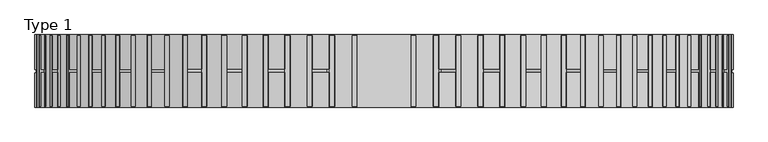
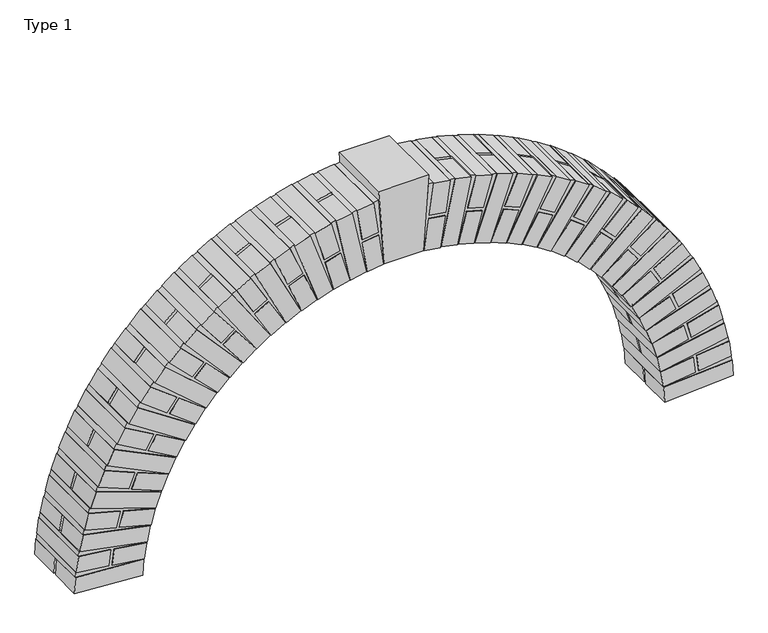
"""IFC4 building model written with IfcOpenShell, lengths in millimetres: proxy geometry, 00_GM_toog : Type 1."""

from ifc_helpers import new_model, si_unit, frame, origin, place, context, project, spatial, polyline, outline, extrude, source, transform, mapped, element, save


def type_1_de08efeb(model_context):
    return source(origin(), model_context, "Body", "SweptSolid", [
        extrude(outline(polyline([(-41.1694034, 158.0337642), (-39.7015699, 142.0396534), (-138.7087275, 127.9832407), (-131.6805212, 78.4796619), (-32.6733636, 92.5360745), (-30.4140828, 76.622699), (-231.7563983, 61.2874572), (-232.3621237, 64.1855221), (-141.8118024, 77.0412864), (-148.8400087, 126.5448652), (-241.2763519, 113.4213355), (-241.8346853, 116.0926555), (-41.1694034, 158.0337642)])), frame((0.0, 2.5, 0.0), z_axis=(0.0, 1.0, 0.0), x_axis=(0.0, 0.0, 1.0)), (0.0, 0.0, 1.0), 205.0),
        extrude(outline(polyline([(0.0, 50.0), (210.0, 50.0), (210.0, 0.0), (0.0, 0.0), (0.0, 50.0)])), frame((78.4796619, 210.0, -131.6805212), z_axis=(0.14056412625055034, 0.0, 0.9900715764082006), x_axis=(0.0, -1.0, 0.0)), (0.0, 0.0, 1.0), 100.0),
        extrude(outline(polyline([(0.0, 50.0), (210.0, 50.0), (210.0, 0.0), (0.0, 0.0), (0.0, 50.0)])), frame((62.9848738, 210.0, -240.81896), z_axis=(0.14056412625055034, 0.0, 0.9900715764082006), x_axis=(0.0, -1.0, 0.0)), (0.0, 0.0, 1.0), 100.0),
        extrude(outline(polyline([(210.0, 50.0000001), (210.0, 0.0), (110.0, 0.0), (110.0, 50.0000001), (210.0, 50.0000001)])), frame((164.0124098, 0.0, -256.956928), z_axis=(0.2045892845565526, 0.0, 0.9788479067989255), x_axis=(0.0, 1.0, 0.0)), (0.0, 0.0, 1.0), 210.0),
        extrude(outline(polyline([(100.0, 50.0000001), (100.0, 0.0), (0.0, 0.0), (0.0, 50.0000001), (100.0, 50.0000001)])), frame((164.0124098, 0.0, -256.956928), z_axis=(0.2045892845565526, 0.0, 0.9788479067989255), x_axis=(0.0, 1.0, 0.0)), (0.0, 0.0, 1.0), 210.0),
        extrude(outline(polyline([(-70.1056799, 286.4239748), (-66.5764443, 270.7551966), (-162.925286, 243.9801952), (-149.5377853, 195.8057743), (-53.1889436, 222.5807757), (-48.8854098, 207.0946701), (-246.5397389, 165.7828815), (-247.5161135, 168.5779444), (-159.3970443, 193.0659212), (-172.784545, 241.2403421), (-262.7389968, 216.2423189), (-263.6389798, 218.8186958), (-70.1056799, 286.4239748)])), frame((0.0, 2.5, 0.0), z_axis=(0.0, 1.0, 0.0), x_axis=(0.0, 0.0, 1.0)), (0.0, 0.0, 1.0), 205.0),
        extrude(outline(polyline([(0.0, 50.0), (210.0, 50.0), (210.0, 0.0), (0.0, 0.0), (0.0, 50.0)])), frame((195.8057743, 210.0, -149.5377853), z_axis=(0.26775001392461106, 0.0, 0.9634884171817379), x_axis=(0.0, -1.0, 0.0)), (0.0, 0.0, 1.0), 100.0),
        extrude(outline(polyline([(0.0, 50.0), (210.0, 50.0), (210.0, 0.0), (0.0, 0.0), (0.0, 50.0)])), frame((166.2909198, 210.0, -255.745886), z_axis=(0.26775001392461106, 0.0, 0.9634884171817379), x_axis=(0.0, -1.0, 0.0)), (0.0, 0.0, 1.0), 100.0),
        extrude(outline(polyline([(210.0, 50.0), (210.0, 0.0), (110.0, 0.0), (110.0, 50.0), (210.0, 50.0)])), frame((264.3731909, 0.0, -284.8468332), z_axis=(0.3297794481680561, 0.0, 0.9440580043439982), x_axis=(0.0, 1.0, 0.0)), (0.0, 0.0, 1.0), 210.0),
        extrude(outline(polyline([(100.0, 50.0), (100.0, 0.0), (0.0, 0.0), (0.0, 50.0), (100.0, 50.0)])), frame((264.3731909, 0.0, -284.8468332), z_axis=(0.3297794481680561, 0.0, 0.9440580043439982), x_axis=(0.0, 1.0, 0.0)), (0.0, 0.0, 1.0), 210.0),
        extrude(outline(polyline([(-115.4447373, 409.978514), (-109.9136834, 394.899603), (-201.9775599, 355.8580528), (-182.4567849, 309.8261146), (-90.3929083, 348.8676647), (-84.1177777, 334.0702796), (-274.7471392, 267.4794077), (-276.077679, 270.1242796), (-191.8775686, 305.8310406), (-211.3983437, 351.8629788), (-297.3522109, 315.4125018), (-298.5786492, 317.8504387), (-115.4447373, 409.978514)])), frame((0.0, 2.5, 0.0), z_axis=(0.0, 1.0, 0.0), x_axis=(0.0, 0.0, 1.0)), (0.0, 0.0, 1.0), 205.0),
        extrude(outline(polyline([(0.0, 49.9999999), (210.0, 49.9999999), (210.0, 0.0), (0.0, 0.0), (0.0, 49.9999999)])), frame((309.8261146, 210.0, -182.4567849), z_axis=(0.39041550103890255, 0.0, 0.9206387655038988), x_axis=(0.0, -1.0, 0.0)), (0.0, 0.0, 1.0), 100.0),
        extrude(outline(polyline([(0.0, 49.9999999), (210.0, 49.9999999), (210.0, 0.0), (0.0, 0.0), (0.0, 49.9999999)])), frame((266.7894905, 210.0, -283.9414452), z_axis=(0.39041550103890255, 0.0, 0.9206387655038988), x_axis=(0.0, -1.0, 0.0)), (0.0, 0.0, 1.0), 100.0),
        extrude(outline(polyline([(210.0, 50.0), (210.0, 0.0), (110.0, 0.0), (110.0, 50.0), (210.0, 50.0)])), frame((360.2705822, 0.0, -325.5140628), z_axis=(0.4494019735925478, 0.0, 0.8933296514339615), x_axis=(0.0, 1.0, 0.0)), (0.0, 0.0, 1.0), 210.0),
        extrude(outline(polyline([(100.0, 50.0), (100.0, 0.0), (0.0, 0.0), (0.0, 50.0), (100.0, 50.0)])), frame((360.2705822, 0.0, -325.5140628), z_axis=(0.4494019735925478, 0.0, 0.8933296514339615), x_axis=(0.0, 1.0, 0.0)), (0.0, 0.0, 1.0), 210.0),
        extrude(outline(polyline([(-176.4211202, 526.6114211), (-168.9816283, 512.3769532), (-255.2062332, 461.7279895), (-229.8817513, 418.6156871), (-143.6571465, 469.2646507), (-135.5163616, 455.4058092), (-315.9023763, 364.6601019), (-317.5646179, 367.1101298), (-238.7050095, 413.4328407), (-264.0294914, 456.5451431), (-344.5316223, 409.2576025), (-346.0638099, 411.5159399), (-176.4211202, 526.6114211)])), frame((0.0, 2.5, 0.0), z_axis=(0.0, 1.0, 0.0), x_axis=(0.0, 0.0, 1.0)), (0.0, 0.0, 1.0), 205.0),
        extrude(outline(polyline([(0.0, 50.0), (210.0, 50.0), (210.0, 0.0), (0.0, 0.0), (0.0, 50.0)])), frame((418.6156871, 210.0, -229.8817513), z_axis=(0.5064896366773486, 0.0, 0.8622460483750839), x_axis=(0.0, -1.0, 0.0)), (0.0, 0.0, 1.0), 100.0),
        extrude(outline(polyline([(0.0, 50.0), (210.0, 50.0), (210.0, 0.0), (0.0, 0.0), (0.0, 50.0)])), frame((362.783877, 210.0, -324.9296144), z_axis=(0.5064896366773486, 0.0, 0.8622460483750839), x_axis=(0.0, -1.0, 0.0)), (0.0, 0.0, 1.0), 100.0),
        extrude(outline(polyline([(210.0, 50.0), (210.0, 0.0), (110.0, 0.0), (110.0, 50.0), (210.0, 50.0)])), frame((450.085556, 0.0, -378.2720354), z_axis=(0.5614372839756181, 0.0, 0.8275192905075271), x_axis=(0.0, 1.0, 0.0)), (0.0, 0.0, 1.0), 210.0),
        extrude(outline(polyline([(100.0, 50.0), (100.0, 0.0), (0.0, 0.0), (0.0, 50.0), (100.0, 50.0)])), frame((450.085556, 0.0, -378.2720354), z_axis=(0.5614372839756181, 0.0, 0.8275192905075271), x_axis=(0.0, 1.0, 0.0)), (0.0, 0.0, 1.0), 210.0),
        extrude(outline(polyline([(-252.0053697, 634.3535926), (-242.7830401, 621.2038872), (-321.7126506, 559.802612), (-291.012013, 520.3378068), (-212.0824025, 581.7390819), (-202.2134034, 569.0527614), (-369.3106297, 455.6842709), (-371.2765096, 457.8980911), (-299.0887834, 514.0546895), (-329.7894209, 553.5194948), (-403.4807049, 496.1932421), (-405.2927741, 498.2338527), (-252.0053697, 634.3535926)])), frame((0.0, 2.5, 0.0), z_axis=(0.0, 1.0, 0.0), x_axis=(0.0, 0.0, 1.0)), (0.0, 0.0, 1.0), 205.0),
        extrude(outline(polyline([(0.0, 50.0), (210.0, 50.0), (210.0, 0.0), (0.0, 0.0), (0.0, 50.0)])), frame((520.3378068, 210.0, -291.012013), z_axis=(0.6140127511464796, 0.0, 0.7892961050388704), x_axis=(0.0, -1.0, 0.0)), (0.0, 0.0, 1.0), 100.0),
        extrude(outline(polyline([(0.0, 49.9999999), (210.0, 49.9999999), (210.0, 0.0), (0.0, 0.0), (0.0, 49.9999999)])), frame((452.6534144, 210.0, -378.0183939), z_axis=(0.6140127511464796, 0.0, 0.7892961050388704), x_axis=(0.0, -1.0, 0.0)), (0.0, 0.0, 1.0), 100.0),
        extrude(outline(polyline([(210.0, 50.0), (210.0, 0.0), (110.0, 0.0), (110.0, 50.0), (210.0, 50.0)])), frame((532.3017739, 0.0, -442.2300429), z_axis=(0.663993896764768, 0.0, 0.7477379922533953), x_axis=(0.0, 1.0, 0.0)), (0.0, 0.0, 1.0), 210.0),
        extrude(outline(polyline([(100.0, 50.0), (100.0, 0.0), (0.0, 0.0), (0.0, 50.0), (100.0, 50.0)])), frame((532.3017739, 0.0, -442.2300429), z_axis=(0.663993896764768, 0.0, 0.7477379922533953), x_axis=(0.0, 1.0, 0.0)), (0.0, 0.0, 1.0), 210.0),
        extrude(outline(polyline([(-340.9214032, 731.3860267), (-330.0719357, 719.5430891), (-400.37399, 648.426135), (-364.8155129, 613.2751079), (-294.5134586, 684.3920619), (-283.0828629, 673.0924447), (-434.0702126, 539.0151613), (-436.306541, 540.9553981), (-372.009436, 605.997797), (-407.5679131, 641.1488242), (-473.2042264, 574.7516936), (-475.2655843, 576.5401261), (-340.9214032, 731.3860267)])), frame((0.0, 2.5, 0.0), z_axis=(0.0, 1.0, 0.0), x_axis=(0.0, 0.0, 1.0)), (0.0, 0.0, 1.0), 205.0),
        extrude(outline(polyline([(0.0, 100.0), (210.0, 100.0), (210.0, 0.0), (0.0, 0.0), (0.0, 100.0)])), frame((648.426135, 210.0, -400.37399), z_axis=(-0.7030205431424774, 0.0, 0.7111695409110659), x_axis=(0.0, -1.0, 0.0)), (0.0, 0.0, 1.0), 50.0),
        extrude(outline(polyline([(0.0, 100.0), (210.0, 100.0), (210.0, 0.0), (0.0, 0.0), (0.0, 100.0)])), frame((570.0318701, 210.0, -477.8699674), z_axis=(-0.7030205431424774, 0.0, 0.7111695409110659), x_axis=(0.0, -1.0, 0.0)), (0.0, 0.0, 1.0), 50.0),
        extrude(outline(polyline([(0.0, 100.0), (210.0, 100.0), (210.0, 0.0), (0.0, 0.0), (0.0, 100.0)])), frame((605.5311866, 110.0, -516.3082875), z_axis=(-0.655332697498948, 0.0, 0.755340357447391), x_axis=(0.755340357447391, 0.0, 0.655332697498948)), (0.0, 0.0, 1.0), 50.0),
        extrude(outline(polyline([(0.0, 100.0), (210.0, 100.0), (210.0, 0.0), (0.0, 0.0), (0.0, 100.0)])), frame((605.5311866, 0.0, -516.3082875), z_axis=(-0.655332697498948, 0.0, 0.755340357447391), x_axis=(0.755340357447391, 0.0, 0.655332697498948)), (0.0, 0.0, 1.0), 50.0),
        extrude(outline(polyline([(-441.6680589, 816.0705332), (-429.3746242, 805.7343067), (-489.8622187, 726.1023351), (-450.0462329, 695.8585378), (-389.5586384, 775.4905094), (-376.7594277, 765.7683658), (-509.0877943, 613.2459049), (-511.5568156, 614.8798014), (-456.2358544, 687.7098957), (-496.0518402, 717.9536929), (-552.5250506, 643.6066616), (-554.8008954, 645.1127218), (-441.6680589, 816.0705332)])), frame((0.0, 2.5, 0.0), z_axis=(0.0, 1.0, 0.0), x_axis=(0.0, 0.0, 1.0)), (0.0, 0.0, 1.0), 205.0),
        extrude(outline(polyline([(0.0, 99.9999999), (210.0, 99.9999999), (210.0, 0.0), (0.0, 0.0), (0.0, 99.9999999)])), frame((726.1023351, 210.0, -489.8622187), z_axis=(-0.6048759456103062, 0.0, 0.7963197162082813), x_axis=(0.0, -1.0, 0.0)), (0.0, 0.0, 1.0), 50.0),
        extrude(outline(polyline([(0.0, 100.0), (210.0, 100.0), (210.0, 0.0), (0.0, 0.0), (0.0, 100.0)])), frame((638.3217213, 210.0, -556.5394348), z_axis=(-0.6048759456103062, 0.0, 0.7963197162082813), x_axis=(0.0, -1.0, 0.0)), (0.0, 0.0, 1.0), 50.0),
        extrude(outline(polyline([(0.0, 100.0), (210.0000001, 100.0), (210.0000001, 0.0), (0.0, 0.0), (0.0, 100.0)])), frame((668.537468, 110.0, -599.2561127), z_axis=(-0.5518634769235881, 0.0, 0.8339344715490591), x_axis=(0.8339344715490591, 0.0, 0.5518634769235881)), (0.0, 0.0, 1.0), 50.0),
        extrude(outline(polyline([(0.0, 100.0), (210.0000001, 100.0), (210.0000001, 0.0), (0.0, 0.0), (0.0, 100.0)])), frame((668.537468, 0.0, -599.2561127), z_axis=(-0.5518634769235881, 0.0, 0.8339344715490591), x_axis=(0.8339344715490591, 0.0, 0.5518634769235881)), (0.0, 0.0, 1.0), 50.0),
        extrude(outline(polyline([(-552.5444398, 886.9773907), (-539.0145868, 878.322381), (-588.6665147, 791.5198116), (-545.26523, 766.6938476), (-495.6133021, 853.496417), (-481.6615645, 845.5158852), (-593.0968596, 677.1232704), (-595.7568893, 678.4232417), (-550.346051, 757.811447), (-593.7473357, 782.637411), (-640.1040109, 701.5956733), (-642.5559196, 702.7939348), (-552.5444398, 886.9773907)])), frame((0.0, 2.5, 0.0), z_axis=(0.0, 1.0, 0.0), x_axis=(0.0, 0.0, 1.0)), (0.0, 0.0, 1.0), 205.0),
        extrude(outline(polyline([(0.0, 100.0), (210.0, 100.0), (210.0, 0.0), (0.0, 0.0), (0.0, 100.0)])), frame((791.5198116, 210.0, -588.6665147), z_axis=(-0.4965192792791466, 0.0, 0.8680256939193199), x_axis=(0.0, -1.0, 0.0)), (0.0, 0.0, 1.0), 50.0),
        extrude(outline(polyline([(0.0, 100.0), (210.0, 100.0), (210.0, 0.0), (0.0, 0.0), (0.0, 100.0)])), frame((695.8348416, 210.0, -643.3992636), z_axis=(-0.4965192792791466, 0.0, 0.8680256939193199), x_axis=(0.0, -1.0, 0.0)), (0.0, 0.0, 1.0), 50.0),
        extrude(outline(polyline([(0.0, 100.0), (210.0, 100.0), (210.0, 0.0), (0.0, 0.0), (0.0, 100.0)])), frame((720.2568887, 110.0, -689.6731173), z_axis=(-0.4390771925190386, 0.0, 0.898449341370786), x_axis=(0.898449341370786, 0.0, 0.4390771925190386)), (0.0, 0.0, 1.0), 50.0),
        extrude(outline(polyline([(0.0, 100.0), (210.0, 100.0), (210.0, 0.0), (0.0, 0.0), (0.0, 100.0)])), frame((720.2568887, 0.0, -689.6731173), z_axis=(-0.4390771925190386, 0.0, 0.898449341370786), x_axis=(0.898449341370786, 0.0, 0.4390771925190386)), (0.0, 0.0, 1.0), 50.0),
        extrude(outline(polyline([(-671.6786294, 942.9094849), (-657.1407815, 936.0818137), (-695.1187735, 843.5741269), (-648.8649301, 824.5851308), (-610.8869381, 917.0928176), (-596.0182196, 910.9886322), (-684.6790905, 729.5688217), (-687.4852197, 730.5129205), (-652.7511715, 815.1189325), (-699.0050149, 834.1079286), (-734.4625191, 747.7397054), (-737.0490965, 748.6099379), (-671.6786294, 942.9094849)])), frame((0.0, 2.5, 0.0), z_axis=(0.0, 1.0, 0.0), x_axis=(0.0, 0.0, 1.0)), (0.0, 0.0, 1.0), 205.0),
        extrude(outline(polyline([(0.0, 100.0), (210.0, 100.0), (210.0, 0.0), (0.0, 0.0), (0.0, 100.0)])), frame((843.5741269, 210.0, -695.1187735), z_axis=(-0.3797799204689407, 0.0, 0.9250768681621031), x_axis=(0.0, -1.0, 0.0)), (0.0, 0.0, 1.0), 50.0),
        extrude(outline(polyline([(0.0, 100.0), (210.0, 100.0), (210.0, 0.0), (0.0, 0.0), (0.0, 100.0)])), frame((741.6002418, 210.0, -736.983007), z_axis=(-0.3797799204689407, 0.0, 0.9250768681621031), x_axis=(0.0, -1.0, 0.0)), (0.0, 0.0, 1.0), 50.0),
        extrude(outline(polyline([(0.0, 100.0), (210.0, 100.0), (210.0, 0.0), (0.0, 0.0), (0.0, 100.0)])), frame((759.8162739, 110.0, -786.0327989), z_axis=(-0.31887800546790185, 0.0, 0.947795767889271), x_axis=(0.947795767889271, 0.0, 0.31887800546790185)), (0.0, 0.0, 1.0), 50.0),
        extrude(outline(polyline([(0.0, 100.0), (210.0, 100.0), (210.0, 0.0), (0.0, 0.0), (0.0, 100.0)])), frame((759.8162739, 0.0, -786.0327989), z_axis=(-0.31887800546790185, 0.0, 0.947795767889271), x_axis=(0.947795767889271, 0.0, 0.31887800546790185)), (0.0, 0.0, 1.0), 50.0),
        extrude(outline(polyline([(-797.0592953, 982.922519), (-781.7588937, 978.0374573), (-807.4217707, 881.3864524), (-759.0962683, 868.5550139), (-733.4333913, 965.2060188), (-717.8987192, 961.0812362), (-782.2883121, 769.697125), (-785.1931651, 770.2694122), (-761.722319, 858.664835), (-810.0478215, 871.4962734), (-834.0075286, 781.2597121), (-836.6851057, 781.7872235), (-797.0592953, 982.922519)])), frame((0.0, 2.5, 0.0), z_axis=(0.0, 1.0, 0.0), x_axis=(0.0, 0.0, 1.0)), (0.0, 0.0, 1.0), 205.0),
        extrude(outline(polyline([(0.0, 100.0), (210.0, 100.0), (210.0, 0.0), (0.0, 0.0), (0.0, 100.0)])), frame((881.3864524, 210.0, -807.4217707), z_axis=(-0.25662876977901194, 0.0, 0.9665100488467313), x_axis=(0.0, -1.0, 0.0)), (0.0, 0.0, 1.0), 50.0),
        extrude(outline(polyline([(0.0, 99.9999999), (210.0, 99.9999999), (210.0, 0.0), (0.0, 0.0), (0.0, 99.9999999)])), frame((774.8452686, 210.0, -835.7106985), z_axis=(-0.25662876977901194, 0.0, 0.9665100488467313), x_axis=(0.0, -1.0, 0.0)), (0.0, 0.0, 1.0), 50.0),
        extrude(outline(polyline([(0.0, 100.0), (210.0, 100.0), (210.0, 0.0), (0.0, 0.0), (0.0, 100.0)])), frame((786.5477461, 110.0, -886.7083253), z_axis=(-0.19329522835345544, 0.0, 0.9811406396107469), x_axis=(0.9811406396107469, 0.0, 0.19329522835345544)), (0.0, 0.0, 1.0), 50.0),
        extrude(outline(polyline([(0.0, 100.0), (210.0, 100.0), (210.0, 0.0), (0.0, 0.0), (0.0, 100.0)])), frame((786.5477461, 0.0, -886.7083253), z_axis=(-0.19329522835345544, 0.0, 0.9811406396107469), x_axis=(0.9811406396107469, 0.0, 0.19329522835345544)), (0.0, 0.0, 1.0), 50.0),
        extrude(outline(polyline([(-926.5696466, 1006.3409563), (-910.7650067, 1003.4809782), (-923.6795044, 904.3184059), (-874.0982183, 897.861157), (-861.1837205, 997.0237294), (-845.2453653, 994.947988), (-884.2765962, 796.8306977), (-887.2311307, 797.0215114), (-875.419743, 887.7139725), (-925.0010292, 894.1712214), (-937.0584296, 801.5897779), (-939.781801, 801.7656623), (-926.5696466, 1006.3409563)])), frame((0.0, 2.5, 0.0), z_axis=(0.0, 1.0, 0.0), x_axis=(0.0, 0.0, 1.0)), (0.0, 0.0, 1.0), 205.0),
        extrude(outline(polyline([(0.0, 100.0), (210.0, 100.0), (210.0, 0.0), (0.0, 0.0), (0.0, 100.0)])), frame((904.3184059, 210.0, -923.6795044), z_axis=(-0.12914497754199947, 0.0, 0.9916257231313015), x_axis=(0.0, -1.0, 0.0)), (0.0, 0.0, 1.0), 50.0),
        extrude(outline(polyline([(0.0, 100.0000001), (210.0, 100.0000001), (210.0, 0.0), (0.0, 0.0), (0.0, 100.0000001)])), frame((795.008649, 210.0, -937.9155269), z_axis=(-0.12914497754199947, 0.0, 0.9916257231313015), x_axis=(0.0, -1.0, 0.0)), (0.0, 0.0, 1.0), 50.0),
        extrude(outline(polyline([(0.0, 100.0), (210.0, 100.0), (210.0, 0.0), (0.0, 0.0), (0.0, 100.0)])), frame((800.0, 110.0, -990.0), z_axis=(-0.06444906444906115, 0.0, 0.9979209979209982), x_axis=(0.9979209979209982, 0.0, 0.06444906444906115)), (0.0, 0.0, 1.0), 50.0),
        extrude(outline(polyline([(0.0, 100.0), (210.0, 100.0), (210.0, 0.0), (0.0, 0.0), (0.0, 100.0)])), frame((800.0, 0.0, -990.0), z_axis=(-0.06444906444906115, 0.0, 0.9979209979209982), x_axis=(0.9979209979209982, 0.0, 0.06444906444906115)), (0.0, 0.0, 1.0), 50.0),
        extrude(outline(polyline([(-41.1694034, -158.0337642), (-241.8346853, -116.0926555), (-241.2763519, -113.4213355), (-148.8400087, -126.5448652), (-141.8118024, -77.0412864), (-232.3621237, -64.1855221), (-231.7563983, -61.2874572), (-30.4140828, -76.622699), (-32.6733636, -92.5360745), (-131.6805212, -78.4796619), (-138.7087275, -127.9832407), (-39.7015699, -142.0396534), (-41.1694034, -158.0337642)])), frame((0.0, 2.5, 0.0), z_axis=(0.0, 1.0, 0.0), x_axis=(0.0, 0.0, 1.0)), (0.0, 0.0, 1.0), 205.0),
        extrude(outline(polyline([(0.0, -50.0), (0.0, 0.0), (210.0, 0.0), (210.0, -50.0), (0.0, -50.0)])), frame((-78.4796619, 210.0, -131.6805212), z_axis=(-0.14056412625055034, 0.0, 0.9900715764082006), x_axis=(0.0, -1.0, 0.0)), (0.0, 0.0, 1.0), 100.0),
        extrude(outline(polyline([(0.0, -50.0), (0.0, 0.0), (210.0, 0.0), (210.0, -50.0), (0.0, -50.0)])), frame((-62.9848738, 210.0, -240.81896), z_axis=(-0.14056412625055034, 0.0, 0.9900715764082006), x_axis=(0.0, -1.0, 0.0)), (0.0, 0.0, 1.0), 100.0),
        extrude(outline(polyline([(210.0, -50.0000001), (110.0, -50.0000001), (110.0, 0.0), (210.0, 0.0), (210.0, -50.0000001)])), frame((-164.0124098, 0.0, -256.956928), z_axis=(-0.2045892845565526, 0.0, 0.9788479067989255), x_axis=(0.0, 1.0, 0.0)), (0.0, 0.0, 1.0), 210.0),
        extrude(outline(polyline([(100.0, -50.0000001), (0.0, -50.0000001), (0.0, 0.0), (100.0, 0.0), (100.0, -50.0000001)])), frame((-164.0124098, 0.0, -256.956928), z_axis=(-0.2045892845565526, 0.0, 0.9788479067989255), x_axis=(0.0, 1.0, 0.0)), (0.0, 0.0, 1.0), 210.0),
        extrude(outline(polyline([(-70.1056799, -286.4239748), (-263.6389798, -218.8186958), (-262.7389968, -216.2423189), (-172.784545, -241.2403421), (-159.3970443, -193.0659212), (-247.5161135, -168.5779444), (-246.5397389, -165.7828815), (-48.8854098, -207.0946701), (-53.1889436, -222.5807757), (-149.5377853, -195.8057743), (-162.925286, -243.9801952), (-66.5764443, -270.7551966), (-70.1056799, -286.4239748)])), frame((0.0, 2.5, 0.0), z_axis=(0.0, 1.0, 0.0), x_axis=(0.0, 0.0, 1.0)), (0.0, 0.0, 1.0), 205.0),
        extrude(outline(polyline([(0.0, -50.0), (0.0, 0.0), (210.0, 0.0), (210.0, -50.0), (0.0, -50.0)])), frame((-195.8057743, 210.0, -149.5377853), z_axis=(-0.26775001392461106, 0.0, 0.9634884171817379), x_axis=(0.0, -1.0, 0.0)), (0.0, 0.0, 1.0), 100.0),
        extrude(outline(polyline([(0.0, -50.0), (0.0, 0.0), (210.0, 0.0), (210.0, -50.0), (0.0, -50.0)])), frame((-166.2909198, 210.0, -255.745886), z_axis=(-0.26775001392461106, 0.0, 0.9634884171817379), x_axis=(0.0, -1.0, 0.0)), (0.0, 0.0, 1.0), 100.0),
        extrude(outline(polyline([(210.0, -50.0), (110.0, -50.0), (110.0, 0.0), (210.0, 0.0), (210.0, -50.0)])), frame((-264.3731909, 0.0, -284.8468332), z_axis=(-0.3297794481680561, 0.0, 0.9440580043439982), x_axis=(0.0, 1.0, 0.0)), (0.0, 0.0, 1.0), 210.0),
        extrude(outline(polyline([(100.0, -50.0), (0.0, -50.0), (0.0, 0.0), (100.0, 0.0), (100.0, -50.0)])), frame((-264.3731909, 0.0, -284.8468332), z_axis=(-0.3297794481680561, 0.0, 0.9440580043439982), x_axis=(0.0, 1.0, 0.0)), (0.0, 0.0, 1.0), 210.0),
        extrude(outline(polyline([(-115.4447373, -409.978514), (-298.5786492, -317.8504387), (-297.3522109, -315.4125018), (-211.3983437, -351.8629788), (-191.8775686, -305.8310406), (-276.077679, -270.1242796), (-274.7471392, -267.4794077), (-84.1177777, -334.0702796), (-90.3929083, -348.8676647), (-182.4567849, -309.8261146), (-201.9775599, -355.8580528), (-109.9136834, -394.899603), (-115.4447373, -409.978514)])), frame((0.0, 2.5, 0.0), z_axis=(0.0, 1.0, 0.0), x_axis=(0.0, 0.0, 1.0)), (0.0, 0.0, 1.0), 205.0),
        extrude(outline(polyline([(0.0, -49.9999999), (0.0, 0.0), (210.0, 0.0), (210.0, -49.9999999), (0.0, -49.9999999)])), frame((-309.8261146, 210.0, -182.4567849), z_axis=(-0.39041550103890255, 0.0, 0.9206387655038988), x_axis=(0.0, -1.0, 0.0)), (0.0, 0.0, 1.0), 100.0),
        extrude(outline(polyline([(0.0, -49.9999999), (0.0, 0.0), (210.0, 0.0), (210.0, -49.9999999), (0.0, -49.9999999)])), frame((-266.7894905, 210.0, -283.9414452), z_axis=(-0.39041550103890255, 0.0, 0.9206387655038988), x_axis=(0.0, -1.0, 0.0)), (0.0, 0.0, 1.0), 100.0),
        extrude(outline(polyline([(210.0, -50.0), (110.0, -50.0), (110.0, 0.0), (210.0, 0.0), (210.0, -50.0)])), frame((-360.2705822, 0.0, -325.5140628), z_axis=(-0.4494019735925478, 0.0, 0.8933296514339615), x_axis=(0.0, 1.0, 0.0)), (0.0, 0.0, 1.0), 210.0),
        extrude(outline(polyline([(100.0, -50.0), (0.0, -50.0), (0.0, 0.0), (100.0, 0.0), (100.0, -50.0)])), frame((-360.2705822, 0.0, -325.5140628), z_axis=(-0.4494019735925478, 0.0, 0.8933296514339615), x_axis=(0.0, 1.0, 0.0)), (0.0, 0.0, 1.0), 210.0),
        extrude(outline(polyline([(-176.4211202, -526.6114211), (-346.0638099, -411.5159399), (-344.5316223, -409.2576025), (-264.0294914, -456.5451431), (-238.7050095, -413.4328407), (-317.5646179, -367.1101298), (-315.9023763, -364.6601019), (-135.5163616, -455.4058092), (-143.6571465, -469.2646507), (-229.8817513, -418.6156871), (-255.2062332, -461.7279895), (-168.9816283, -512.3769532), (-176.4211202, -526.6114211)])), frame((0.0, 2.5, 0.0), z_axis=(0.0, 1.0, 0.0), x_axis=(0.0, 0.0, 1.0)), (0.0, 0.0, 1.0), 205.0),
        extrude(outline(polyline([(0.0, -50.0), (0.0, 0.0), (210.0, 0.0), (210.0, -50.0), (0.0, -50.0)])), frame((-418.6156871, 210.0, -229.8817513), z_axis=(-0.5064896366773486, 0.0, 0.8622460483750839), x_axis=(0.0, -1.0, 0.0)), (0.0, 0.0, 1.0), 100.0),
        extrude(outline(polyline([(0.0, -50.0), (0.0, 0.0), (210.0, 0.0), (210.0, -50.0), (0.0, -50.0)])), frame((-362.783877, 210.0, -324.9296144), z_axis=(-0.5064896366773486, 0.0, 0.8622460483750839), x_axis=(0.0, -1.0, 0.0)), (0.0, 0.0, 1.0), 100.0),
        extrude(outline(polyline([(210.0, -50.0), (110.0, -50.0), (110.0, 0.0), (210.0, 0.0), (210.0, -50.0)])), frame((-450.085556, 0.0, -378.2720354), z_axis=(-0.5614372839756181, 0.0, 0.8275192905075271), x_axis=(0.0, 1.0, 0.0)), (0.0, 0.0, 1.0), 210.0),
        extrude(outline(polyline([(100.0, -50.0), (0.0, -50.0), (0.0, 0.0), (100.0, 0.0), (100.0, -50.0)])), frame((-450.085556, 0.0, -378.2720354), z_axis=(-0.5614372839756181, 0.0, 0.8275192905075271), x_axis=(0.0, 1.0, 0.0)), (0.0, 0.0, 1.0), 210.0),
        extrude(outline(polyline([(-252.0053697, -634.3535926), (-405.2927741, -498.2338527), (-403.4807049, -496.1932421), (-329.7894209, -553.5194948), (-299.0887834, -514.0546895), (-371.2765096, -457.8980911), (-369.3106297, -455.6842709), (-202.2134034, -569.0527614), (-212.0824025, -581.7390819), (-291.012013, -520.3378068), (-321.7126506, -559.802612), (-242.7830401, -621.2038872), (-252.0053697, -634.3535926)])), frame((0.0, 2.5, 0.0), z_axis=(0.0, 1.0, 0.0), x_axis=(0.0, 0.0, 1.0)), (0.0, 0.0, 1.0), 205.0),
        extrude(outline(polyline([(0.0, -50.0), (0.0, 0.0), (210.0, 0.0), (210.0, -50.0), (0.0, -50.0)])), frame((-520.3378068, 210.0, -291.012013), z_axis=(-0.6140127511464796, 0.0, 0.7892961050388704), x_axis=(0.0, -1.0, 0.0)), (0.0, 0.0, 1.0), 100.0),
        extrude(outline(polyline([(0.0, -49.9999999), (0.0, 0.0), (210.0, 0.0), (210.0, -49.9999999), (0.0, -49.9999999)])), frame((-452.6534144, 210.0, -378.0183939), z_axis=(-0.6140127511464796, 0.0, 0.7892961050388704), x_axis=(0.0, -1.0, 0.0)), (0.0, 0.0, 1.0), 100.0),
        extrude(outline(polyline([(210.0, -50.0), (110.0, -50.0), (110.0, 0.0), (210.0, 0.0), (210.0, -50.0)])), frame((-532.3017739, 0.0, -442.2300429), z_axis=(-0.663993896764768, 0.0, 0.7477379922533953), x_axis=(0.0, 1.0, 0.0)), (0.0, 0.0, 1.0), 210.0),
        extrude(outline(polyline([(100.0, -50.0), (0.0, -50.0), (0.0, 0.0), (100.0, 0.0), (100.0, -50.0)])), frame((-532.3017739, 0.0, -442.2300429), z_axis=(-0.663993896764768, 0.0, 0.7477379922533953), x_axis=(0.0, 1.0, 0.0)), (0.0, 0.0, 1.0), 210.0),
        extrude(outline(polyline([(-340.9214032, -731.3860267), (-475.2655843, -576.5401261), (-473.2042264, -574.7516936), (-407.5679131, -641.1488242), (-372.009436, -605.997797), (-436.306541, -540.9553981), (-434.0702126, -539.0151613), (-283.0828629, -673.0924447), (-294.5134586, -684.3920619), (-364.8155129, -613.2751079), (-400.37399, -648.426135), (-330.0719357, -719.5430891), (-340.9214032, -731.3860267)])), frame((0.0, 2.5, 0.0), z_axis=(0.0, 1.0, 0.0), x_axis=(0.0, 0.0, 1.0)), (0.0, 0.0, 1.0), 205.0),
        extrude(outline(polyline([(0.0, -100.0), (0.0, 0.0), (210.0, 0.0), (210.0, -100.0), (0.0, -100.0)])), frame((-648.426135, 210.0, -400.37399), z_axis=(0.7030205431424774, 0.0, 0.7111695409110659), x_axis=(0.0, -1.0, 0.0)), (0.0, 0.0, 1.0), 50.0),
        extrude(outline(polyline([(0.0, -100.0), (0.0, 0.0), (210.0, 0.0), (210.0, -100.0), (0.0, -100.0)])), frame((-570.0318701, 210.0, -477.8699674), z_axis=(0.7030205431424774, 0.0, 0.7111695409110659), x_axis=(0.0, -1.0, 0.0)), (0.0, 0.0, 1.0), 50.0),
        extrude(outline(polyline([(0.0, -100.0), (0.0, 0.0), (210.0, 0.0), (210.0, -100.0), (0.0, -100.0)])), frame((-605.5311866, 110.0, -516.3082875), z_axis=(0.655332697498948, 0.0, 0.755340357447391), x_axis=(-0.755340357447391, 0.0, 0.655332697498948)), (0.0, 0.0, 1.0), 50.0),
        extrude(outline(polyline([(0.0, -100.0), (0.0, 0.0), (210.0, 0.0), (210.0, -100.0), (0.0, -100.0)])), frame((-605.5311866, 0.0, -516.3082875), z_axis=(0.655332697498948, 0.0, 0.755340357447391), x_axis=(-0.755340357447391, 0.0, 0.655332697498948)), (0.0, 0.0, 1.0), 50.0),
        extrude(outline(polyline([(-441.6680589, -816.0705332), (-554.8008954, -645.1127218), (-552.5250506, -643.6066616), (-496.0518402, -717.9536929), (-456.2358544, -687.7098957), (-511.5568156, -614.8798014), (-509.0877943, -613.2459049), (-376.7594277, -765.7683658), (-389.5586384, -775.4905094), (-450.0462329, -695.8585378), (-489.8622187, -726.1023351), (-429.3746242, -805.7343067), (-441.6680589, -816.0705332)])), frame((0.0, 2.5, 0.0), z_axis=(0.0, 1.0, 0.0), x_axis=(0.0, 0.0, 1.0)), (0.0, 0.0, 1.0), 205.0),
        extrude(outline(polyline([(0.0, -99.9999999), (0.0, 0.0), (210.0, 0.0), (210.0, -99.9999999), (0.0, -99.9999999)])), frame((-726.1023351, 210.0, -489.8622187), z_axis=(0.6048759456103062, 0.0, 0.7963197162082813), x_axis=(0.0, -1.0, 0.0)), (0.0, 0.0, 1.0), 50.0),
        extrude(outline(polyline([(0.0, -100.0), (0.0, 0.0), (210.0, 0.0), (210.0, -100.0), (0.0, -100.0)])), frame((-638.3217213, 210.0, -556.5394348), z_axis=(0.6048759456103062, 0.0, 0.7963197162082813), x_axis=(0.0, -1.0, 0.0)), (0.0, 0.0, 1.0), 50.0),
        extrude(outline(polyline([(0.0, -100.0), (0.0, 0.0), (210.0000001, 0.0), (210.0000001, -100.0), (0.0, -100.0)])), frame((-668.537468, 110.0, -599.2561127), z_axis=(0.5518634769235881, 0.0, 0.8339344715490591), x_axis=(-0.8339344715490591, 0.0, 0.5518634769235881)), (0.0, 0.0, 1.0), 50.0),
        extrude(outline(polyline([(0.0, -100.0), (0.0, 0.0), (210.0000001, 0.0), (210.0000001, -100.0), (0.0, -100.0)])), frame((-668.537468, 0.0, -599.2561127), z_axis=(0.5518634769235881, 0.0, 0.8339344715490591), x_axis=(-0.8339344715490591, 0.0, 0.5518634769235881)), (0.0, 0.0, 1.0), 50.0),
        extrude(outline(polyline([(-552.5444398, -886.9773907), (-642.5559196, -702.7939348), (-640.1040109, -701.5956733), (-593.7473357, -782.637411), (-550.346051, -757.811447), (-595.7568893, -678.4232417), (-593.0968596, -677.1232704), (-481.6615645, -845.5158852), (-495.6133021, -853.496417), (-545.26523, -766.6938476), (-588.6665147, -791.5198116), (-539.0145868, -878.322381), (-552.5444398, -886.9773907)])), frame((0.0, 2.5, 0.0), z_axis=(0.0, 1.0, 0.0), x_axis=(0.0, 0.0, 1.0)), (0.0, 0.0, 1.0), 205.0),
        extrude(outline(polyline([(0.0, -100.0), (0.0, 0.0), (210.0, 0.0), (210.0, -100.0), (0.0, -100.0)])), frame((-791.5198116, 210.0, -588.6665147), z_axis=(0.4965192792791466, 0.0, 0.8680256939193199), x_axis=(0.0, -1.0, 0.0)), (0.0, 0.0, 1.0), 50.0),
        extrude(outline(polyline([(0.0, -100.0), (0.0, 0.0), (210.0, 0.0), (210.0, -100.0), (0.0, -100.0)])), frame((-695.8348416, 210.0, -643.3992636), z_axis=(0.4965192792791466, 0.0, 0.8680256939193199), x_axis=(0.0, -1.0, 0.0)), (0.0, 0.0, 1.0), 50.0),
        extrude(outline(polyline([(0.0, -100.0), (0.0, 0.0), (210.0, 0.0), (210.0, -100.0), (0.0, -100.0)])), frame((-720.2568887, 110.0, -689.6731173), z_axis=(0.4390771925190386, 0.0, 0.898449341370786), x_axis=(-0.898449341370786, 0.0, 0.4390771925190386)), (0.0, 0.0, 1.0), 50.0),
        extrude(outline(polyline([(0.0, -100.0), (0.0, 0.0), (210.0, 0.0), (210.0, -100.0), (0.0, -100.0)])), frame((-720.2568887, 0.0, -689.6731173), z_axis=(0.4390771925190386, 0.0, 0.898449341370786), x_axis=(-0.898449341370786, 0.0, 0.4390771925190386)), (0.0, 0.0, 1.0), 50.0),
        extrude(outline(polyline([(-671.6786294, -942.9094849), (-737.0490965, -748.6099379), (-734.4625191, -747.7397054), (-699.0050149, -834.1079286), (-652.7511715, -815.1189325), (-687.4852197, -730.5129205), (-684.6790905, -729.5688217), (-596.0182196, -910.9886322), (-610.8869381, -917.0928176), (-648.8649301, -824.5851308), (-695.1187735, -843.5741269), (-657.1407815, -936.0818137), (-671.6786294, -942.9094849)])), frame((0.0, 2.5, 0.0), z_axis=(0.0, 1.0, 0.0), x_axis=(0.0, 0.0, 1.0)), (0.0, 0.0, 1.0), 205.0),
        extrude(outline(polyline([(0.0, -100.0), (0.0, 0.0), (210.0, 0.0), (210.0, -100.0), (0.0, -100.0)])), frame((-843.5741269, 210.0, -695.1187735), z_axis=(0.3797799204689407, 0.0, 0.9250768681621031), x_axis=(0.0, -1.0, 0.0)), (0.0, 0.0, 1.0), 50.0),
        extrude(outline(polyline([(0.0, -100.0), (0.0, 0.0), (210.0, 0.0), (210.0, -100.0), (0.0, -100.0)])), frame((-741.6002418, 210.0, -736.983007), z_axis=(0.3797799204689407, 0.0, 0.9250768681621031), x_axis=(0.0, -1.0, 0.0)), (0.0, 0.0, 1.0), 50.0),
        extrude(outline(polyline([(0.0, -100.0), (0.0, 0.0), (210.0, 0.0), (210.0, -100.0), (0.0, -100.0)])), frame((-759.8162739, 110.0, -786.0327989), z_axis=(0.31887800546790185, 0.0, 0.947795767889271), x_axis=(-0.947795767889271, 0.0, 0.31887800546790185)), (0.0, 0.0, 1.0), 50.0),
        extrude(outline(polyline([(0.0, -100.0), (0.0, 0.0), (210.0, 0.0), (210.0, -100.0), (0.0, -100.0)])), frame((-759.8162739, 0.0, -786.0327989), z_axis=(0.31887800546790185, 0.0, 0.947795767889271), x_axis=(-0.947795767889271, 0.0, 0.31887800546790185)), (0.0, 0.0, 1.0), 50.0),
        extrude(outline(polyline([(-797.0592953, -982.922519), (-836.6851057, -781.7872235), (-834.0075286, -781.2597121), (-810.0478215, -871.4962734), (-761.722319, -858.664835), (-785.1931651, -770.2694122), (-782.2883121, -769.697125), (-717.8987192, -961.0812362), (-733.4333913, -965.2060188), (-759.0962683, -868.5550139), (-807.4217707, -881.3864524), (-781.7588937, -978.0374573), (-797.0592953, -982.922519)])), frame((0.0, 2.5, 0.0), z_axis=(0.0, 1.0, 0.0), x_axis=(0.0, 0.0, 1.0)), (0.0, 0.0, 1.0), 205.0),
        extrude(outline(polyline([(0.0, -100.0), (0.0, 0.0), (210.0, 0.0), (210.0, -100.0), (0.0, -100.0)])), frame((-881.3864524, 210.0, -807.4217707), z_axis=(0.25662876977901194, 0.0, 0.9665100488467313), x_axis=(0.0, -1.0, 0.0)), (0.0, 0.0, 1.0), 50.0),
        extrude(outline(polyline([(0.0, -99.9999999), (0.0, 0.0), (210.0, 0.0), (210.0, -99.9999999), (0.0, -99.9999999)])), frame((-774.8452686, 210.0, -835.7106985), z_axis=(0.25662876977901194, 0.0, 0.9665100488467313), x_axis=(0.0, -1.0, 0.0)), (0.0, 0.0, 1.0), 50.0),
        extrude(outline(polyline([(0.0, -100.0), (0.0, 0.0), (210.0, 0.0), (210.0, -100.0), (0.0, -100.0)])), frame((-786.5477461, 110.0, -886.7083253), z_axis=(0.19329522835345544, 0.0, 0.9811406396107469), x_axis=(-0.9811406396107469, 0.0, 0.19329522835345544)), (0.0, 0.0, 1.0), 50.0),
        extrude(outline(polyline([(0.0, -100.0), (0.0, 0.0), (210.0, 0.0), (210.0, -100.0), (0.0, -100.0)])), frame((-786.5477461, 0.0, -886.7083253), z_axis=(0.19329522835345544, 0.0, 0.9811406396107469), x_axis=(-0.9811406396107469, 0.0, 0.19329522835345544)), (0.0, 0.0, 1.0), 50.0),
        extrude(outline(polyline([(-926.5696466, -1006.3409563), (-939.781801, -801.7656623), (-937.0584296, -801.5897779), (-925.0010292, -894.1712214), (-875.419743, -887.7139725), (-887.2311307, -797.0215114), (-884.2765962, -796.8306977), (-845.2453653, -994.947988), (-861.1837205, -997.0237294), (-874.0982183, -897.861157), (-923.6795044, -904.3184059), (-910.7650067, -1003.4809782), (-926.5696466, -1006.3409563)])), frame((0.0, 2.5, 0.0), z_axis=(0.0, 1.0, 0.0), x_axis=(0.0, 0.0, 1.0)), (0.0, 0.0, 1.0), 205.0),
        extrude(outline(polyline([(0.0, -100.0), (0.0, 0.0), (210.0, 0.0), (210.0, -100.0), (0.0, -100.0)])), frame((-904.3184059, 210.0, -923.6795044), z_axis=(0.12914497754199947, 0.0, 0.9916257231313015), x_axis=(0.0, -1.0, 0.0)), (0.0, 0.0, 1.0), 50.0),
        extrude(outline(polyline([(0.0, -100.0000001), (0.0, 0.0), (210.0, 0.0), (210.0, -100.0000001), (0.0, -100.0000001)])), frame((-795.008649, 210.0, -937.9155269), z_axis=(0.12914497754199947, 0.0, 0.9916257231313015), x_axis=(0.0, -1.0, 0.0)), (0.0, 0.0, 1.0), 50.0),
        extrude(outline(polyline([(0.0, -100.0), (0.0, 0.0), (210.0, 0.0), (210.0, -100.0), (0.0, -100.0)])), frame((-800.0, 110.0, -990.0), z_axis=(0.06444906444906115, 0.0, 0.9979209979209982), x_axis=(-0.9979209979209982, 0.0, 0.06444906444906115)), (0.0, 0.0, 1.0), 50.0),
        extrude(outline(polyline([(0.0, -100.0), (0.0, 0.0), (210.0, 0.0), (210.0, -100.0), (0.0, -100.0)])), frame((-800.0, 0.0, -990.0), z_axis=(0.06444906444906115, 0.0, 0.9979209979209982), x_axis=(-0.9979209979209982, 0.0, 0.06444906444906115)), (0.0, 0.0, 1.0), 50.0),
        extrude(outline(polyline([(0.0, 77.2240527), (0.0, -77.2240527), (-240.0, -59.431631), (-240.0, 59.431631), (0.0, 77.2240527)])), frame((0.0, 0.0, 0.0), z_axis=(0.0, 1.0, 0.0), x_axis=(0.0, 0.0, 1.0)), (0.0, 0.0, 1.0), 210.0),
    ])


if __name__ == "__main__":
    model = new_model("IFC4")
    model_context = context("Model", 3, world=origin())
    ifc_project = project(units=[si_unit("LENGTHUNIT", "METRE", prefix="MILLI")], contexts=[model_context])
    site = spatial("IfcSite", under=ifc_project)
    building = spatial("IfcBuilding", under=site)
    placement = place(None, origin())
    type_1_shape = type_1_de08efeb(model_context)
    element("IfcBuildingElementProxy", 1, Name="00_GM_toog : Type 1", ObjectType="00_GM_toog : Type 1", at=placement, inside=building, context=model_context, shape_type="MappedRepresentation", body=[
        mapped(type_1_shape, transform((0.0, 0.0, 0.0), x_axis=(1.0, 0.0, 0.0), y_axis=(0.0, 1.0, 0.0), z_axis=(0.0, 0.0, 1.0))),
    ])
    save(model, "model.ifc")

# Revit data of these elements
# Type "00_GM_toog : Type 1"
#   straal_hart_rollaag [instance default] = 1935 mm
#   straal_buitenlijn [instance default] = 2040 mm
#   straal [instance default] = 1830 mm
#   stootvoegbreedte_onderzijde [instance default] = 5 mm
#   offset [instance default] = -2070 mm
#   kop_voeg [instance default] = 55 mm
#   hoek_sluitsteen_half [instance default] = 2.80637°
#   hoek_kop [instance default] = 1.72149°
#   halve_breedte_tov_balk [instance default] = 200 mm
#   half_b [instance default] = 1800 mm
#   h_toog [instance default] = 1500 mm
#   h_steen [instance default] = 210 mm
#   h_sluitsteen [instance default] = 240 mm
#   h_kop [instance default] = 50 mm
#   dekdikte [instance default] = 240 mm
#   breedte [instance default] = 4000 mm
#   b_sluitsteen_bovenzijde [instance default] = 200 mm
#   apothema [instance default] = 330 mm
#   aantal_strekken [instance default] = 14
#   materiaal_voeg [instance default] = none
#   materiaal_strek [instance default] = none
#   materiaal_sluitsteen [instance default] = none
#   materiaal_koppen [instance default] = none
#   Default Elevation = 0
# Element 1 (IfcBuildingElementProxy, "00_GM_toog : Type 1")
#   straal_hart_rollaag = 906.667 mm
#   straal_buitenlijn = 1011.667 mm
#   straal = 801.667 mm
#   offset = -1041.667 mm
#   hoek_sluitsteen_half = 4.23987°
#   hoek_kop = 3.92475°
#   half_b = 800 mm
#   h_toog = 750 mm
#   breedte = 2000 mm
#   b_sluitsteen_bovenzijde = 150 mm
#   apothema = 51.667 mm
